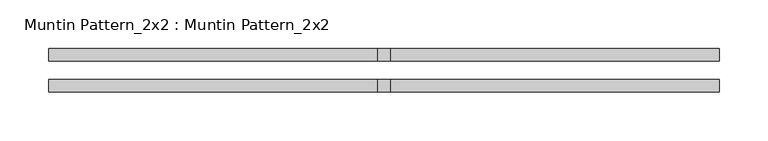
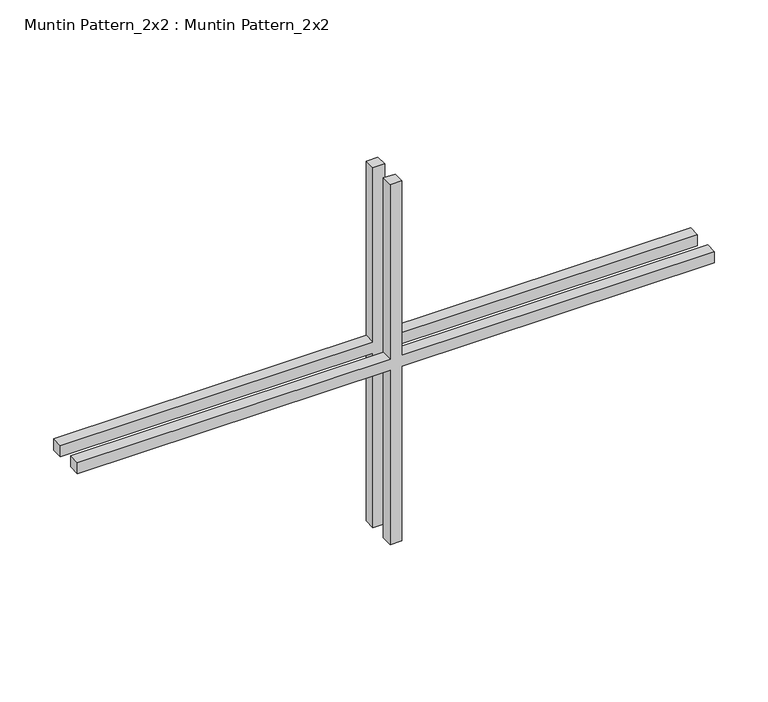
"""IFC4 building model written with IfcOpenShell, lengths in millimetres: proxy geometry, Muntin Pattern_2x2 : Muntin Pattern_2x2."""

from ifc_helpers import new_model, si_unit, frame, origin, place, context, project, spatial, polyline, outline, extrude, source, transform, mapped, element, save


def muntin_pattern_2x2_muntin_pattern_2x2_e664c3e5(model_context):
    return source(origin(), model_context, "Body", "SweptSolid", [
        extrude(outline(polyline([(211.1375, -6.35), (211.1375, -342.9), (198.4375, -342.9), (198.4375, -6.35), (0.0, -6.35), (0.0, 6.35), (198.4375, 6.35), (198.4375, 342.9), (211.1375, 342.9), (211.1375, 6.35), (409.575, 6.35), (409.575, -6.35), (211.1375, -6.35)])), frame((0.0, 9.525, 0.0), z_axis=(0.0, 1.0, 0.0), x_axis=(0.0, 0.0, 1.0)), (0.0, 0.0, 1.0), 12.7),
        extrude(outline(polyline([(211.1375, -6.35), (211.1375, -342.9), (198.4375, -342.9), (198.4375, -6.35), (0.0, -6.35), (0.0, 6.35), (198.4375, 6.35), (198.4375, 342.9), (211.1375, 342.9), (211.1375, 6.35), (409.575, 6.35), (409.575, -6.35), (211.1375, -6.35)])), frame((0.0, -22.225, 0.0), z_axis=(0.0, 1.0, 0.0), x_axis=(0.0, 0.0, 1.0)), (0.0, 0.0, 1.0), 12.7),
    ])


if __name__ == "__main__":
    model = new_model("IFC4")
    model_context = context("Model", 3, world=origin())
    ifc_project = project(units=[si_unit("LENGTHUNIT", "METRE", prefix="MILLI")], contexts=[model_context])
    site = spatial("IfcSite", under=ifc_project)
    building = spatial("IfcBuilding", under=site)
    placement = place(None, origin())
    muntin_pattern_2x2_muntin_pattern_2x2_shape = muntin_pattern_2x2_muntin_pattern_2x2_e664c3e5(model_context)
    element("IfcBuildingElementProxy", 1, Name="Muntin Pattern_2x2 : Muntin Pattern_2x2", ObjectType="Muntin Pattern_2x2 : Muntin Pattern_2x2", at=placement, inside=building, context=model_context, shape_type="MappedRepresentation", body=[
        mapped(muntin_pattern_2x2_muntin_pattern_2x2_shape, transform((0.0, 0.0, 0.0), x_axis=(1.0, 0.0, 0.0), y_axis=(0.0, 1.0, 0.0), z_axis=(0.0, 0.0, 1.0))),
    ])
    save(model, "model.ifc")

# Revit data of these elements
# Type "Muntin Pattern_2x2 : Muntin Pattern_2x2"
#   Width [instance default] = 4' - 0"
#   Thickness = 0' - 0 1/2"
#   Height [instance default] = 4' - 0"
#   Distance = 0' - 0 3/4"
#   Interior Material [instance default] = none
#   Exterior Material [instance default] = none
# Element 1 (IfcBuildingElementProxy, "Muntin Pattern_2x2 : Muntin Pattern_2x2")
#   Width = 2' - 3"
#   Height = 1' - 4 1/8"
#   Interior Material = Wood - Stained
#   Exterior Material = Clad - White
#   Materials on its faces: "Clad - White", "Wood - Stained"
# Materials
#   "Clad - White": class "Wood", colour RGB 242 242 238, transparency 0, Cost = 0
#   "Wood - Stained": class "Wood", colour RGB 224 178 126, transparency 0, Cost = 0
